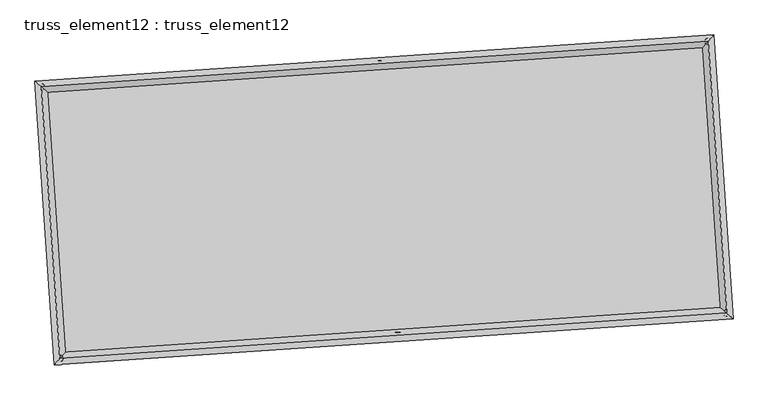
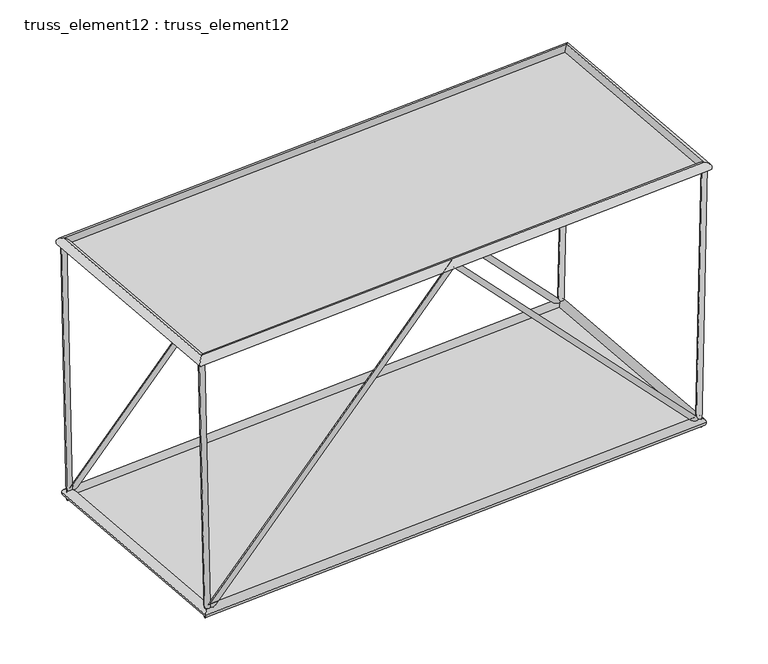
"""IFC4 building model written with IfcOpenShell, lengths in millimetres: plate geometry, truss_element12 : truss_element12."""

from ifc_helpers import new_model, si_unit, frame, origin, origin_with_axes, place, context, project, spatial, polyline, circle_curve, ellipse_curve, outline, extrude, source, transform, mapped, element, save
from ifc_brep_helpers import plane_surface, cylinder_surface, advanced_brep


def truss_element12_truss_element12_9a917d05(model_context):
    return source(origin(), model_context, "Body", "SolidModel", [
        advanced_brep(
        [(-3777.9297062, 2268.5197435, 4999.8474769), (-3877.0075384, 2255.1602403, 4997.5876475), (-3667.6713064, 2276.0378447, 121.3370365), (-3761.3155765, 2263.0488354, -121.3370365), (1063.300848, 2598.6248518, 5070.8413416), (1063.7552992, 2592.0520766, 4926.6125798), (5795.0902874, 2921.2675864, 121.3427195), (5889.6706896, 2921.1129021, -121.3427195), (5904.5374646, 2928.7303734, 4999.8579637), (6004.5120743, 2928.9434995, 4997.6147547)],
        [
            (0, 1, circle_curve(frame((-3827.4686223, 2261.8399919, 4998.7175622), z_axis=(-0.022595036175344915, -0.0015406696250232525, 0.999743512445738), x_axis=(-0.1335955830397217, 0.991034809561541, -0.0014921225140709302)), 50.0)),
            (1, 0, circle_curve(frame((-3827.4686223, 2261.8399919, 4998.7175622), z_axis=(-0.022595036175344915, -0.0015406696250232525, 0.999743512445738), x_axis=(-0.1335955830397217, 0.991034809561541, -0.0014921225140709302)), 50.0)),
            (0, 2),
            (2, 3, ellipse_curve(frame((-3714.4934414, 2269.54334, 0.0), z_axis=(-0.9299262044326746, -0.06340813289982028, 0.3622384062901093), x_axis=(0.3613992433762671, 0.02464244059868928, 0.9320854773079569)), 130.4614748, 50.0)),
            (3, 1),
            (3, 2, ellipse_curve(frame((-3714.4934414, 2269.54334, 0.0), z_axis=(-0.9299262044326746, -0.06340813289982028, 0.3622384062901093), x_axis=(0.3613992433762671, 0.02464244059868928, 0.9320854773079569)), 130.4614748, 50.0)),
            (2, 4),
            (4, 5, ellipse_curve(frame((1063.5280736, 2595.3384642, 4998.7269607), z_axis=(-0.9976833951339081, -0.06802823816454197, -4.3431630552355546e-05), x_axis=(4.333101666675271e-05, 2.9545773097502304e-06, -0.9999999990568467)), 72.2714089, 50.0)),
            (5, 3),
            (5, 4, ellipse_curve(frame((1063.5280736, 2595.3384642, 4998.7269607), z_axis=(-0.9976833951339081, -0.06802823816454197, -4.3431630552355546e-05), x_axis=(4.333101666675271e-05, 2.9545773097502304e-06, -0.9999999990568467)), 72.2714089, 50.0)),
            (4, 6),
            (6, 7, ellipse_curve(frame((5842.3804885, 2921.1902443, 0.0), z_axis=(-0.9298803947541625, -0.06340500931198113, -0.36235653194883977), x_axis=(-0.3615170953846328, -0.02465047647914223, 0.9320395612601481)), 130.4740125, 50.0)),
            (7, 5),
            (7, 6, ellipse_curve(frame((5842.3804885, 2921.1902443, 0.0), z_axis=(-0.9298803947541625, -0.06340500931198113, -0.36235653194883977), x_axis=(-0.3615170953846328, -0.02465047647914223, 0.9320395612601481)), 130.4740125, 50.0)),
            (8, 9, circle_curve(frame((5954.5247694, 2928.8369365, 4998.7363592), z_axis=(0.022428856188337464, 0.0015293384434184449, 0.9997472718312406), x_axis=(-0.002165029131322687, 0.9999965594182461, -0.0014811483824928716)), 50.0)),
            (9, 8, circle_curve(frame((5954.5247694, 2928.8369365, 4998.7363592), z_axis=(0.022428856188337464, 0.0015293384434184449, 0.9997472718312406), x_axis=(-0.002165029131322687, 0.9999965594182461, -0.0014811483824928716)), 50.0)),
            (6, 8),
            (9, 7),
        ],
        [
            plane_surface(frame((-3827.4686223, 2311.8399326, 4998.7946154), z_axis=(-0.02259503617534488, -0.0015406696250278634, 0.999743512445738), x_axis=(0.9997446995809655, -3.482037556779006e-05, 0.022595009345131704))),
            cylinder_surface(frame((-3827.4686223, 2261.8399919, 4998.7175622), z_axis=(-0.022595036175344915, -0.0015406696250232525, 0.999743512445738), x_axis=(-0.1335955830397217, 0.991034809561541, -0.0014921225140709302)), 50.0),
            cylinder_surface(frame((-3714.4934414, 2269.54334, 0.0), z_axis=(-0.690202519980209, -0.04706228613204369, -0.7220842212906988), x_axis=(-0.02041638033504215, 0.9987520691595456, -0.04557933482995593)), 50.0),
            cylinder_surface(frame((1063.5280736, 2595.3384642, 4998.7269607), z_axis=(-0.6902650946631379, -0.047066552861803786, 0.7220241261144925), x_axis=(-0.11534052877108418, 0.9922795523181616, -0.04558346711336914)), 50.0),
            plane_surface(frame((5954.5247694, 2878.836995, 4998.8128453), z_axis=(0.02242885618833652, 0.0015293384434182575, 0.9997472718312408), x_axis=(0.9997484415642183, -3.430994296671486e-05, -0.022428829945962292))),
            cylinder_surface(frame((5842.3804885, 2921.1902443, 0.0), z_axis=(-0.022428856188337468, -0.0015293384434184453, -0.9997472718312408), x_axis=(-0.002165029131322687, 0.9999965594182461, -0.0014811483824928716)), 50.0),
        ],
        [
            (0, [[1, 2]]),
            (1, [[-1, 3, 4, 5]]),
            (1, [[-2, -5, 6, -3]]),
            (2, [[-4, 7, 8, 9]]),
            (2, [[-6, -9, 10, -7]]),
            (3, [[-8, 11, 12, 13]]),
            (3, [[-10, -13, 14, -11]]),
            (4, [[15, 16]]),
            (5, [[-12, 17, -16, 18]]),
            (5, [[-14, -18, -15, -17]]),
        ],
    ),
        advanced_brep(
        [(-3505.8167532, -1722.2138408, 4999.8474769), (-3604.8945855, -1735.573344, 4997.5876475), (-3395.5583535, -1714.6957396, 121.3370365), (-3489.2026235, -1727.6847489, -121.3370365), (1335.4138009, -1392.1087325, 5070.8413416), (1335.8682521, -1398.6815077, 4926.6125798), (6067.2032403, -1069.4659979, 121.3427195), (6161.7836425, -1069.6206822, -121.3427195), (6176.6504175, -1062.0032109, 4999.8579637), (6276.6250272, -1061.7900848, 4997.6147547)],
        [
            (0, 1, circle_curve(frame((-3555.3556694, -1728.8935924, 4998.7175622), z_axis=(-0.022595036175344977, -0.0015406696250231744, 0.9997435124457379), x_axis=(-0.13359558303972127, 0.9910348095615411, -0.0014921225140710067)), 50.0)),
            (1, 0, circle_curve(frame((-3555.3556694, -1728.8935924, 4998.7175622), z_axis=(-0.022595036175344977, -0.0015406696250231744, 0.9997435124457379), x_axis=(-0.13359558303972127, 0.9910348095615411, -0.0014921225140710067)), 50.0)),
            (0, 2),
            (2, 3, ellipse_curve(frame((-3442.3804885, -1721.1902443, 0.0), z_axis=(-0.9299262044326748, -0.06340813289981997, 0.36223840629010895), x_axis=(0.36139924337626683, 0.024642440598689214, 0.932085477307957)), 130.4614748, 50.0)),
            (3, 1),
            (3, 2, ellipse_curve(frame((-3442.3804885, -1721.1902443, 0.0), z_axis=(-0.9299262044326748, -0.06340813289981997, 0.36223840629010895), x_axis=(0.36139924337626683, 0.024642440598689214, 0.932085477307957)), 130.4614748, 50.0)),
            (2, 4),
            (4, 5, ellipse_curve(frame((1335.6410265, -1395.3951201, 4998.7269607), z_axis=(-0.9976833951339081, -0.06802823816454182, -4.343163055259626e-05), x_axis=(4.3331016666752704e-05, 2.9545773098367193e-06, -0.9999999990568467)), 72.2714089, 50.0)),
            (5, 3),
            (5, 4, ellipse_curve(frame((1335.6410265, -1395.3951201, 4998.7269607), z_axis=(-0.9976833951339081, -0.06802823816454182, -4.343163055259626e-05), x_axis=(4.3331016666752704e-05, 2.9545773098367193e-06, -0.9999999990568467)), 72.2714089, 50.0)),
            (4, 6),
            (6, 7, ellipse_curve(frame((6114.4934414, -1069.54334, 0.0), z_axis=(-0.9298803947541623, -0.06340500931198094, -0.36235653194884), x_axis=(-0.3615170953846332, -0.024650476479142282, 0.932039561260148)), 130.4740125, 50.0)),
            (7, 5),
            (7, 6, ellipse_curve(frame((6114.4934414, -1069.54334, 0.0), z_axis=(-0.9298803947541623, -0.06340500931198094, -0.36235653194884), x_axis=(-0.3615170953846332, -0.024650476479142282, 0.932039561260148)), 130.4740125, 50.0)),
            (8, 9, circle_curve(frame((6226.6377224, -1061.8966478, 4998.7363592), z_axis=(0.022428856188337426, 0.0015293384434183564, 0.9997472718312407), x_axis=(-0.0021650291313227497, 0.9999965594182461, -0.0014811483824927816)), 50.0)),
            (9, 8, circle_curve(frame((6226.6377224, -1061.8966478, 4998.7363592), z_axis=(0.022428856188337426, 0.0015293384434183564, 0.9997472718312407), x_axis=(-0.0021650291313227497, 0.9999965594182461, -0.0014811483824927816)), 50.0)),
            (6, 8),
            (9, 7),
        ],
        [
            plane_surface(frame((-3555.3556694, -1678.8936517, 4998.7946154), z_axis=(-0.02259503617534488, -0.0015406696250278551, 0.999743512445738), x_axis=(0.9997446995809655, -3.482037556779006e-05, 0.022595009345131704))),
            cylinder_surface(frame((-3555.3556694, -1728.8935924, 4998.7175622), z_axis=(-0.02259503617534498, -0.0015406696250231749, 0.9997435124457381), x_axis=(-0.13359558303972127, 0.9910348095615411, -0.0014921225140710067)), 50.0),
            cylinder_surface(frame((-3442.3804885, -1721.1902443, 0.0), z_axis=(-0.6902025199802089, -0.047062286132043524, -0.7220842212906992), x_axis=(-0.020416380335042027, 0.9987520691595456, -0.04557933482995579)), 50.0),
            cylinder_surface(frame((1335.6410265, -1395.3951201, 4998.7269607), z_axis=(-0.6902650946631379, -0.04706655286180374, 0.7220241261144924), x_axis=(-0.1153405287710841, 0.9922795523181616, -0.045583467113369115)), 50.0),
            plane_surface(frame((6226.6377224, -1111.8965893, 4998.8128453), z_axis=(0.022428856188336517, 0.0015293384434182454, 0.9997472718312408), x_axis=(0.9997484415642183, -3.430994296627077e-05, -0.022428829945962292))),
            cylinder_surface(frame((6114.4934414, -1069.54334, 0.0), z_axis=(-0.022428856188337426, -0.0015293384434183564, -0.9997472718312407), x_axis=(-0.0021650291313227497, 0.9999965594182461, -0.0014811483824927816)), 50.0),
        ],
        [
            (0, [[1, 2]]),
            (1, [[-1, 3, 4, 5]]),
            (1, [[-2, -5, 6, -3]]),
            (2, [[-4, 7, 8, 9]]),
            (2, [[-6, -9, 10, -7]]),
            (3, [[-8, 11, 12, 13]]),
            (3, [[-10, -13, 14, -11]]),
            (4, [[15, 16]]),
            (5, [[-12, 17, -16, 18]]),
            (5, [[-14, -18, -15, -17]]),
        ],
    ),
        advanced_brep(
        [(-3555.3507869, -1728.8881809, 4908.7175624), (-3555.3605519, -1728.8990038, 5088.7175621), (-3827.4741942, 2261.8446905, 5088.7175621), (-3827.4630504, 2261.8352933, 4908.7175624), (5954.5293077, 2928.8423245, 5088.736359), (5954.5202312, 2928.8315485, 4908.7363593), (6226.6429499, -1061.9013699, 5088.736359), (6226.6324948, -1061.8919257, 4908.7363593)],
        [
            (0, 1, ellipse_curve(frame((-3555.3556694, -1728.8935924, 4998.7175622), z_axis=(-0.7535719234041632, 0.6573654662781673, -1.3556177535734114e-06), x_axis=(-0.6573654662767825, -0.7535719234053712, -1.35561775357338e-06)), 127.2792206, 90.0)),
            (1, 2),
            (2, 3, ellipse_curve(frame((-3827.4686223, 2261.8399919, 4998.7175622), z_axis=(-0.6573654662767824, -0.7535719234053713, -1.3556177535733527e-06), x_axis=(0.7535719234041632, -0.6573654662781673, 1.3556177535733842e-06)), 127.2792206, 90.0)),
            (3, 0),
            (1, 0, ellipse_curve(frame((-3555.3556694, -1728.8935924, 4998.7175622), z_axis=(-0.7535719234041632, 0.6573654662781673, -1.3556177535734114e-06), x_axis=(-0.6573654662767825, -0.7535719234053712, -1.35561775357338e-06)), 127.2792206, 90.0)),
            (3, 2, ellipse_curve(frame((-3827.4686223, 2261.8399919, 4998.7175622), z_axis=(-0.6573654662767824, -0.7535719234053713, -1.3556177535733527e-06), x_axis=(0.7535719234041632, -0.6573654662781673, 1.3556177535733842e-06)), 127.2792206, 90.0)),
            (2, 4),
            (4, 5, ellipse_curve(frame((5954.5247694, 2928.8369365, 4998.7363592), z_axis=(-0.7535719234041632, 0.6573654662781673, -1.3556177535733563e-06), x_axis=(-0.6573654662767825, -0.7535719234053713, -1.3556177535733807e-06)), 127.2792206, 90.0)),
            (5, 3),
            (5, 4, ellipse_curve(frame((5954.5247694, 2928.8369365, 4998.7363592), z_axis=(-0.7535719234041632, 0.6573654662781673, -1.3556177535733563e-06), x_axis=(-0.6573654662767825, -0.7535719234053713, -1.3556177535733807e-06)), 127.2792206, 90.0)),
            (4, 6),
            (6, 7, ellipse_curve(frame((6226.6377224, -1061.8966478, 4998.7363592), z_axis=(0.6573654662767825, 0.7535719234053713, 1.355617753573408e-06), x_axis=(-0.7535719234041632, 0.6573654662781673, -1.3556177535733834e-06)), 127.2792206, 90.0)),
            (7, 5),
            (7, 6, ellipse_curve(frame((6226.6377224, -1061.8966478, 4998.7363592), z_axis=(0.6573654662767825, 0.7535719234053713, 1.355617753573408e-06), x_axis=(-0.7535719234041632, 0.6573654662781673, -1.3556177535733834e-06)), 127.2792206, 90.0)),
            (6, 1),
            (0, 7),
        ],
        [
            cylinder_surface(frame((-3555.3556694, -1728.8935924, 4998.7175622), z_axis=(0.06802823822870384, -0.9976833960748764, 0.0), x_axis=(-0.9976833943843257, -0.06802823811343162, -5.821470713182902e-05)), 90.0),
            cylinder_surface(frame((-3827.4686223, 2261.8399919, 4998.7175622), z_axis=(-0.997683396073043, -0.06802823822857892, -1.917133012497206e-06), x_axis=(-0.0680282380132191, 0.9976833945011814, -5.629757412236988e-05)), 90.0),
            cylinder_surface(frame((5954.5247694, 2928.8369365, 4998.7363592), z_axis=(-0.06802823822870378, 0.9976833960748763, 0.0), x_axis=(0.9976833945996856, 0.06802823812811613, -5.4380441112910756e-05)), 90.0),
            cylinder_surface(frame((6226.6377224, -1061.8966478, 4998.7363592), z_axis=(0.997683396073043, 0.06802823822857886, 1.9171330124972445e-06), x_axis=(0.06802823822857886, -0.9976833944864969, -5.6297574122369864e-05)), 90.0),
        ],
        [
            (0, [[1, 2, 3, 4]]),
            (0, [[5, -4, 6, -2]]),
            (1, [[-3, 7, 8, 9]]),
            (1, [[-6, -9, 10, -7]]),
            (2, [[-8, 11, 12, 13]]),
            (2, [[-10, -13, 14, -11]]),
            (3, [[-12, 15, -1, 16]]),
            (3, [[-14, -16, -5, -15]]),
        ],
    ),
        advanced_brep(
        [(-3358.7115243, -1625.2761972, 0.0), (-3526.0494527, -1817.1042913, 0.0), (-3810.4074885, 2353.2123043, 0.0), (-3618.5793943, 2185.8743758, 0.0), (5926.0494527, 3017.1042913, 0.0), (5758.7115243, 2825.2761972, 0.0), (6210.4074885, -1153.2123043, 0.0), (6018.5793943, -985.8743758, 0.0)],
        [
            (0, 1, ellipse_curve(frame((-3442.3804885, -1721.1902443, 0.0), z_axis=(-0.7535719234054592, 0.6573654662780793, 0.0), x_axis=(-0.6573654662780793, -0.7535719234054592, 0.0)), 127.2792206, 90.0)),
            (1, 2),
            (2, 3, ellipse_curve(frame((-3714.4934414, 2269.54334, 0.0), z_axis=(-0.6573654662780793, -0.7535719234054592, 0.0), x_axis=(0.7535719234054592, -0.6573654662780793, 0.0)), 127.2792206, 90.0)),
            (3, 0),
            (1, 0, ellipse_curve(frame((-3442.3804885, -1721.1902443, 0.0), z_axis=(-0.7535719234054592, 0.6573654662780793, 0.0), x_axis=(-0.6573654662780793, -0.7535719234054592, 0.0)), 127.2792206, 90.0)),
            (3, 2, ellipse_curve(frame((-3714.4934414, 2269.54334, 0.0), z_axis=(-0.6573654662780793, -0.7535719234054592, 0.0), x_axis=(0.7535719234054592, -0.6573654662780793, 0.0)), 127.2792206, 90.0)),
            (2, 4),
            (4, 5, ellipse_curve(frame((5842.3804885, 2921.1902443, 0.0), z_axis=(-0.753571923405459, 0.6573654662780795, 0.0), x_axis=(-0.6573654662780796, -0.753571923405459, 0.0)), 127.2792206, 90.0)),
            (5, 3),
            (5, 4, ellipse_curve(frame((5842.3804885, 2921.1902443, 0.0), z_axis=(-0.753571923405459, 0.6573654662780795, 0.0), x_axis=(-0.6573654662780796, -0.753571923405459, 0.0)), 127.2792206, 90.0)),
            (4, 6),
            (6, 7, ellipse_curve(frame((6114.4934414, -1069.54334, 0.0), z_axis=(0.6573654662780796, 0.7535719234054591, 0.0), x_axis=(-0.7535719234054591, 0.6573654662780795, 0.0)), 127.2792206, 90.0)),
            (7, 5),
            (7, 6, ellipse_curve(frame((6114.4934414, -1069.54334, 0.0), z_axis=(0.6573654662780796, 0.7535719234054591, 0.0), x_axis=(-0.7535719234054591, 0.6573654662780795, 0.0)), 127.2792206, 90.0)),
            (6, 1),
            (0, 7),
        ],
        [
            cylinder_surface(frame((-3442.3804885, -1721.1902443, 0.0), z_axis=(0.06802823822870326, -0.9976833960748764, 0.0), x_axis=(-0.9976833960748764, -0.06802823822870326, 0.0)), 90.0),
            cylinder_surface(frame((-3714.4934414, 2269.54334, 0.0), z_axis=(-0.9976833960748764, -0.0680282382287031, 0.0), x_axis=(-0.0680282382287031, 0.9976833960748764, 0.0)), 90.0),
            cylinder_surface(frame((5842.3804885, 2921.1902443, 0.0), z_axis=(-0.06802823822870294, 0.9976833960748767, 0.0), x_axis=(0.9976833960748767, 0.06802823822870294, 0.0)), 90.0),
            cylinder_surface(frame((6114.4934414, -1069.54334, 0.0), z_axis=(0.9976833960748767, 0.06802823822870278, 0.0), x_axis=(0.06802823822870278, -0.9976833960748767, 0.0)), 90.0),
        ],
        [
            (0, [[1, 2, 3, 4]]),
            (0, [[5, -4, 6, -2]]),
            (1, [[-3, 7, 8, 9]]),
            (1, [[-6, -9, 10, -7]]),
            (2, [[-8, 11, 12, 13]]),
            (2, [[-10, -13, 14, -11]]),
            (3, [[-12, 15, -1, 16]]),
            (3, [[-14, -16, -5, -15]]),
        ],
    ),
        extrude(outline(polyline([(-3442.3804885, -1721.1902443), (-3714.4934414, 2269.54334), (5842.3804885, 2921.1902443), (6114.4934414, -1069.54334), (-3442.3804885, -1721.1902443)])), origin_with_axes(), (0.0, 0.0, 1.0), 20.0),
        extrude(outline(polyline([(-2000.0, 4902.3535072), (2000.0, 4902.3535072), (2000.0000001, -4902.3535072), (-1999.9999999, -4902.3535073), (-2000.0, 4902.3535072)])), frame((1199.58455, 599.971672, 4998.7269607), z_axis=(-1.9126917746354915e-06, -1.304191812902722e-07, 0.9999999999981624), x_axis=(-0.06802823822870291, 0.9976833960748765, 0.0)), (0.0, 0.0, 1.0), 20.0),
    ])


if __name__ == "__main__":
    model = new_model("IFC4")
    model_context = context("Model", 3, world=origin())
    ifc_project = project(units=[si_unit("LENGTHUNIT", "METRE", prefix="MILLI")], contexts=[model_context])
    site = spatial("IfcSite", under=ifc_project)
    building = spatial("IfcBuilding", under=site)
    placement = place(None, origin())
    truss_element12_truss_element12_shape = truss_element12_truss_element12_9a917d05(model_context)
    element("IfcPlate", 1, ObjectType="truss_element12 : truss_element12", at=placement, inside=building, context=model_context, shape_type="MappedRepresentation", body=[
        mapped(truss_element12_truss_element12_shape, transform((0.0, 0.0, 0.0), x_axis=(1.0, 0.0, 0.0), y_axis=(0.0, 1.0, 0.0), z_axis=(0.0, 0.0, 1.0))),
    ])
    save(model, "model.ifc")

# Revit data of these elements
# Type "truss_element12 : truss_element12"
#   steellbar1 = 90 mm
#   steelbar2 = 50 mm
#   offset1 = 5000 mm
#   M = Default Roof
# Element 1 (IfcPlate, "truss_element12 : truss_element12")
#   Materials on its faces: "Default Roof"
# Materials
#   "Default Roof": class "Miscellaneous", colour RGB 0 127 0, transparency 0, Comments = "Rendering appearance not upgraded Rendering appearance not upgraded ", Cost = 0
